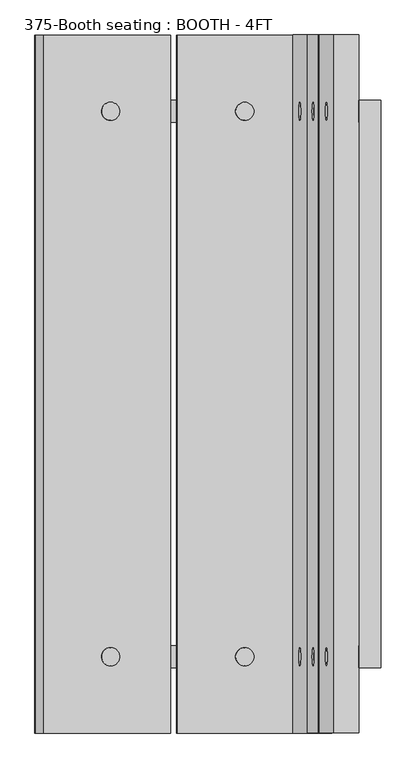
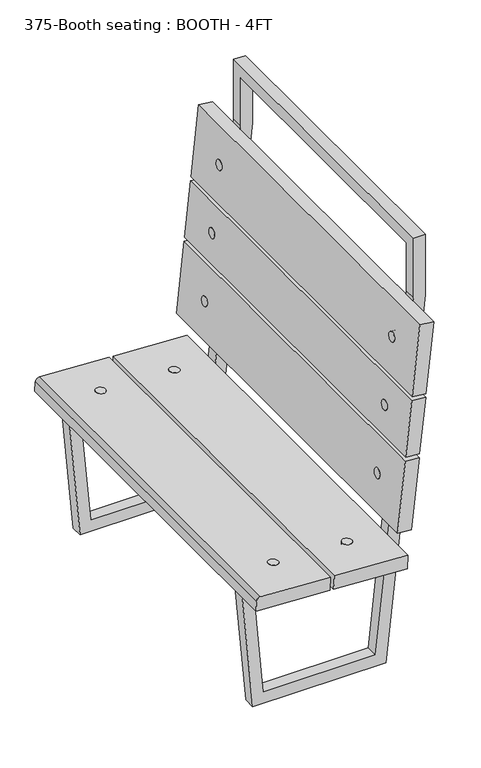
"""IFC4 building model written with IfcOpenShell, lengths in millimetres: furniture geometry, 375-Booth seating : BOOTH - 4FT."""

from ifc_helpers import new_model, si_unit, point, frame, frame_2d, origin, place, context, project, spatial, polyline, circle_curve, trimmed, segment, composite_curve, outline, extrude, faceted_brep, source, transform, mapped, element, save


def furniture_375_booth_seating_booth_4ft_ec9e60ed(model_context):
    return source(origin(), model_context, "Body", "SolidModel", [
        extrude(outline(composite_curve([segment(trimmed(circle_curve(frame_2d((0.0, -15.875)), 15.875), [point((0.0, -31.75))], [point((0.0, 0.0))], False, "CARTESIAN"), True, "CONTINUOUS"), segment(trimmed(circle_curve(frame_2d((0.0, -15.875)), 15.875), [point((0.0, 0.0))], [point((0.0, -31.75))], False, "CARTESIAN"), True, "CONTINUOUS")], self_intersect=False)), frame((476.8022404, 460.375, 403.0070028), z_axis=(0.052335956242943765, 0.0, 0.9986295347545739), x_axis=(-0.9986295347545739, 0.0, 0.052335956242943765)), (0.0, 0.0, 1.0), 44.45),
        extrude(outline(composite_curve([segment(trimmed(circle_curve(frame_2d((-234.95, -15.875)), 15.875), [point((-234.95, -31.75))], [point((-234.95, 0.0))], False, "CARTESIAN"), True, "CONTINUOUS"), segment(trimmed(circle_curve(frame_2d((-234.95, -15.875)), 15.875), [point((-234.95, 0.0))], [point((-234.95, -31.75))], False, "CARTESIAN"), True, "CONTINUOUS")], self_intersect=False)), frame((476.8022404, 460.375, 403.0070028), z_axis=(0.052335956242943765, 0.0, 0.9986295347545739), x_axis=(-0.9986295347545739, 0.0, 0.052335956242943765)), (0.0, 0.0, 1.0), 44.45),
        extrude(outline(composite_curve([segment(trimmed(circle_curve(frame_2d((0.0, 936.625)), 15.875), [point((0.0, 920.75))], [point((0.0, 952.5))], False, "CARTESIAN"), True, "CONTINUOUS"), segment(trimmed(circle_curve(frame_2d((0.0, 936.625)), 15.875), [point((0.0, 952.5))], [point((0.0, 920.75))], False, "CARTESIAN"), True, "CONTINUOUS")], self_intersect=False)), frame((476.8022404, 460.375, 403.0070028), z_axis=(0.052335956242943765, 0.0, 0.9986295347545739), x_axis=(-0.9986295347545739, 0.0, 0.052335956242943765)), (0.0, 0.0, 1.0), 44.45),
        extrude(outline(composite_curve([segment(trimmed(circle_curve(frame_2d((-234.95, 936.625)), 15.875), [point((-234.95, 920.75))], [point((-234.95, 952.5))], False, "CARTESIAN"), True, "CONTINUOUS"), segment(trimmed(circle_curve(frame_2d((-234.95, 936.625)), 15.875), [point((-234.95, 952.5))], [point((-234.95, 920.75))], False, "CARTESIAN"), True, "CONTINUOUS")], self_intersect=False)), frame((476.8022404, 460.375, 403.0070028), z_axis=(0.052335956242943765, 0.0, 0.9986295347545739), x_axis=(-0.9986295347545739, 0.0, 0.052335956242943765)), (0.0, 0.0, 1.0), 44.45),
        extrude(outline(composite_curve([segment(trimmed(circle_curve(frame_2d((0.0, -15.875)), 15.875), [point((0.0, -31.75))], [point((0.0, 0.0))], False, "CARTESIAN"), True, "CONTINUOUS"), segment(trimmed(circle_curve(frame_2d((0.0, -15.875)), 15.875), [point((0.0, 0.0))], [point((0.0, -31.75))], False, "CARTESIAN"), True, "CONTINUOUS")], self_intersect=False)), frame((900.6975371, -492.125, 1069.1522612), z_axis=(-0.9945218953682735, 0.0, 0.10452846326765225), x_axis=(-0.10452846326765225, 0.0, -0.9945218953682735)), (0.0, 0.0, 1.0), 44.45),
        extrude(outline(composite_curve([segment(trimmed(circle_curve(frame_2d((222.2499999, -15.875)), 15.875), [point((222.2499999, -31.75))], [point((222.2499999, 0.0))], False, "CARTESIAN"), True, "CONTINUOUS"), segment(trimmed(circle_curve(frame_2d((222.2499999, -15.875)), 15.875), [point((222.2499999, 0.0))], [point((222.2499999, -31.75))], False, "CARTESIAN"), True, "CONTINUOUS")], self_intersect=False)), frame((900.6975371, -492.125, 1069.1522612), z_axis=(-0.9945218953682735, 0.0, 0.10452846326765225), x_axis=(-0.10452846326765225, 0.0, -0.9945218953682735)), (0.0, 0.0, 1.0), 44.45),
        extrude(outline(composite_curve([segment(trimmed(circle_curve(frame_2d((444.5, -15.875)), 15.875), [point((444.5, -31.75))], [point((444.5, 0.0))], False, "CARTESIAN"), True, "CONTINUOUS"), segment(trimmed(circle_curve(frame_2d((444.5, -15.875)), 15.875), [point((444.5, 0.0))], [point((444.5, -31.75))], False, "CARTESIAN"), True, "CONTINUOUS")], self_intersect=False)), frame((900.6975371, -492.125, 1069.1522612), z_axis=(-0.9945218953682735, 0.0, 0.10452846326765225), x_axis=(-0.10452846326765225, 0.0, -0.9945218953682735)), (0.0, 0.0, 1.0), 44.45),
        extrude(outline(composite_curve([segment(trimmed(circle_curve(frame_2d((0.0, -968.375)), 15.875), [point((0.0, -984.25))], [point((0.0, -952.5))], False, "CARTESIAN"), True, "CONTINUOUS"), segment(trimmed(circle_curve(frame_2d((0.0, -968.375)), 15.875), [point((0.0, -952.5))], [point((0.0, -984.25))], False, "CARTESIAN"), True, "CONTINUOUS")], self_intersect=False)), frame((900.6975371, -492.125, 1069.1522612), z_axis=(-0.9945218953682735, 0.0, 0.10452846326765225), x_axis=(-0.10452846326765225, 0.0, -0.9945218953682735)), (0.0, 0.0, 1.0), 44.45),
        extrude(outline(composite_curve([segment(trimmed(circle_curve(frame_2d((222.2499999, -968.375)), 15.875), [point((222.2499999, -984.25))], [point((222.2499999, -952.5))], False, "CARTESIAN"), True, "CONTINUOUS"), segment(trimmed(circle_curve(frame_2d((222.2499999, -968.375)), 15.875), [point((222.2499999, -952.5))], [point((222.2499999, -984.25))], False, "CARTESIAN"), True, "CONTINUOUS")], self_intersect=False)), frame((900.6975371, -492.125, 1069.1522612), z_axis=(-0.9945218953682735, 0.0, 0.10452846326765225), x_axis=(-0.10452846326765225, 0.0, -0.9945218953682735)), (0.0, 0.0, 1.0), 44.45),
        extrude(outline(composite_curve([segment(trimmed(circle_curve(frame_2d((444.5, -968.375)), 15.875), [point((444.5, -984.25))], [point((444.5, -952.5))], False, "CARTESIAN"), True, "CONTINUOUS"), segment(trimmed(circle_curve(frame_2d((444.5, -968.375)), 15.875), [point((444.5, -952.5))], [point((444.5, -984.25))], False, "CARTESIAN"), True, "CONTINUOUS")], self_intersect=False)), frame((900.6975371, -492.125, 1069.1522612), z_axis=(-0.9945218953682735, 0.0, 0.10452846326765225), x_axis=(-0.10452846326765225, 0.0, -0.9945218953682735)), (0.0, 0.0, 1.0), 44.45),
        faceted_brep([(828.7442542, -457.2, 384.5625035), (914.0084079, -457.2, 1195.7967364), (914.0084079, -457.2, 1358.9), (952.1084079, -457.2, 1358.9), (952.1084079, -457.2, 1193.8), (826.6349718, -457.2, 0.0), (402.5983885, -457.2, 0.0), (366.8356381, -457.2, 408.7701083), (437.5106063, -457.2, 38.1), (792.3295777, -457.2, 38.1), (824.7562543, -457.2, 346.6192193), (408.6106083, -457.2, 368.4284885), (828.7442542, -495.3, 384.5625035), (366.8356381, -495.3, 408.7701083), (402.5983885, -495.3, 0.0), (826.6349718, -495.3, 0.0), (952.1084079, -495.3, 1193.8), (952.1084079, -495.3, 1397.0), (914.0084079, -495.3, 1397.0), (914.0084079, -495.3, 1195.7967364), (437.5106063, -495.3, 38.1), (408.6106083, -495.3, 368.4284885), (824.7562543, -495.3, 346.6192193), (792.3295777, -495.3, 38.1), (914.0084079, 457.2, 1358.9), (952.1084079, 457.2, 1358.9), (828.7442542, 495.3, 384.5625035), (914.0084079, 495.3, 1195.7967364), (914.0084079, 495.3, 1397.0), (952.1084079, 495.3, 1397.0), (952.1084079, 495.3, 1193.8), (826.6349718, 495.3, 0.0), (402.5983885, 495.3, 0.0), (366.8356381, 495.3, 408.7701083), (437.5106063, 495.3, 38.1), (792.3295777, 495.3, 38.1), (824.7562543, 495.3, 346.6192193), (408.6106083, 495.3, 368.4284885), (828.7442542, 457.2, 384.5625035), (366.8356381, 457.2, 408.7701083), (402.5983885, 457.2, 0.0), (826.6349718, 457.2, 0.0), (952.1084079, 457.2, 1193.8), (914.0084079, 457.2, 1195.7967364), (437.5106063, 457.2, 38.1), (408.6106083, 457.2, 368.4284885), (824.7562543, 457.2, 346.6192193), (792.3295777, 457.2, 38.1)], [[[0, 1, 2, 3, 4, 5, 6, 7], [8, 9, 10, 11]], [[12, 13, 14, 15, 16, 17, 18, 19], [20, 21, 22, 23]], [[5, 4, 16, 15]], [[1, 0, 12, 19]], [[0, 7, 13, 12]], [[7, 6, 14, 13]], [[6, 5, 15, 14]], [[8, 11, 21, 20]], [[11, 10, 22, 21]], [[10, 9, 23, 22]], [[9, 8, 20, 23]], [[2, 24, 25, 3]], [[26, 27, 28, 29, 30, 31, 32, 33], [34, 35, 36, 37]], [[38, 39, 40, 41, 42, 25, 24, 43], [44, 45, 46, 47]], [[26, 33, 39, 38]], [[33, 32, 40, 39]], [[32, 31, 41, 40]], [[34, 37, 45, 44]], [[37, 36, 46, 45]], [[36, 35, 47, 46]], [[35, 34, 44, 47]], [[31, 30, 42, 41]], [[27, 26, 38, 43]], [[17, 16, 4, 3, 25, 42, 30, 29]], [[18, 17, 29, 28]], [[19, 18, 28, 27, 43, 24, 2, 1]]]),
        extrude(outline(polyline([(0.0, -44.45), (0.0, 0.0), (1219.2, 0.0), (1219.2, -44.45), (0.0, -44.45)])), frame((841.955154, 609.6, 510.2558191), z_axis=(0.10452846326765272, 0.0, 0.9945218953682734), x_axis=(0.0, -1.0, 0.0)), (0.0, 0.0, 1.0), 234.95),
        extrude(outline(polyline([(0.0, -44.45), (0.0, 0.0), (1219.2, 0.0), (1219.2, -44.45), (0.0, -44.45)])), frame((867.8416279, 609.6, 756.5491664), z_axis=(0.10452846326765385, 0.0, 0.9945218953682733), x_axis=(0.0, -1.0, 0.0)), (0.0, 0.0, 1.0), 184.15),
        extrude(outline(polyline([(0.0, -44.45), (0.0, 0.0), (1219.2, 0.0), (1219.2, -44.45), (0.0, -44.45)])), frame((888.4180559, 609.6, 952.3208015), z_axis=(0.10452846326765004, 0.0, 0.9945218953682737), x_axis=(0.0, -1.0, 0.0)), (0.0, 0.0, 1.0), 234.95),
        extrude(outline(composite_curve([segment(polyline([(441.9125858, 583.7599832), (453.5442521, 361.8145691)]), True, "CONTINUOUS"), segment(trimmed(circle_curve(frame_2d((440.861657, 361.1499024)), 12.7), [point((453.5442521, 361.8145691))], [point((441.5263237, 348.4673073))], False, "CARTESIAN"), True, "CONTINUOUS"), segment(polyline([(441.5263237, 348.4673073), (409.8198359, 346.8056407), (397.4995564, 581.8905778), (441.9125858, 583.7599832)]), True, "CONTINUOUS")], self_intersect=False)), frame((0.0, -609.6, 0.0), z_axis=(0.0, 1.0, 0.0), x_axis=(0.0, 0.0, 1.0)), (0.0, 0.0, 1.0), 1219.2),
        extrude(outline(polyline([(0.0, -234.95), (0.0, 0.0), (1219.2, 0.0), (1219.2, -234.95), (0.0, -234.95)])), frame((828.7442542, 609.6, 384.5625035), z_axis=(0.05233595624294369, 0.0, 0.9986295347545739), x_axis=(0.0, -1.0, 0.0)), (0.0, 0.0, 1.0), 44.45),
    ])


if __name__ == "__main__":
    model = new_model("IFC4")
    model_context = context("Model", 3, world=origin())
    ifc_project = project(units=[si_unit("LENGTHUNIT", "METRE", prefix="MILLI")], contexts=[model_context])
    site = spatial("IfcSite", under=ifc_project)
    building = spatial("IfcBuilding", under=site)
    placement = place(None, origin())
    furniture_375_booth_seating_booth_4ft_shape = furniture_375_booth_seating_booth_4ft_ec9e60ed(model_context)
    element("IfcFurniture", 1, ObjectType="375-Booth seating : BOOTH - 4FT", at=placement, inside=building, context=model_context, shape_type="MappedRepresentation", body=[
        mapped(furniture_375_booth_seating_booth_4ft_shape, transform((0.0, 0.0, 0.0), x_axis=(1.0, 0.0, 0.0), y_axis=(0.0, 1.0, 0.0), z_axis=(0.0, 0.0, 1.0))),
    ])
    save(model, "model.ifc")

# Revit data of these elements
# Type "375-Booth seating : BOOTH - 4FT"
#   tube dim [instance default] = 0' - 1 1/2"
#   seat angle = 3.00°
#   radius of plug = 0' - 0 5/8"
#   plank width_2 = 0' - 7 1/4"
#   plank width_1 = 0' - 9 1/4"
#   plank depth = 0' - 1 3/4"
#   inset = 0' - 6"
#   gap = 0' - 0 1/2"
#   DEPTH = 4' - 0"
#   Seating Count = 2
#   middle support visibility = no
#   Right Bench Visible [instance default] = yes
#   Left Bench Visible [instance default] = yes
#   Material_1 = WOOD-OAKFIRE
#   Material 2 = 1 1/2" SQUARE TUBE STEEL\n- WELDED MITER JOINTS GROUND SMOOTH\n- CLEAR COAT
#   Assembly Code = ""
# Element 1 (IfcFurniture, "375-Booth seating : BOOTH - 4FT")
#   Materials on its faces: "1 1/2\" SQUARE TUBE STEEL\n- WELDED MITER JOINTS GROUND SMOOTH\n- CLEAR COAT", "WOOD-OAKFIRE", "1 1/4\" WOOD PLUG\n(SLIGHTLY DARKER OR STAINED WOOD) - GAL. HEX HEAD THRU BOLT"
# Materials
#   "WOOD-OAKFIRE": class "Wood", colour RGB 198 202 183, transparency 0, Description = "Generic wood", Cost = 0
#   "1 1/2\" SQUARE TUBE STEEL\n- WELDED MITER JOINTS GROUND SMOOTH\n- CLEAR COAT": class "Metal", colour RGB 147 147 147, transparency 0, Cost = 0
#   "1 1/4\" WOOD PLUG\n(SLIGHTLY DARKER OR STAINED WOOD) - GAL. HEX HEAD THRU BOLT": class "Generic", colour RGB 192 192 192, transparency 0, Cost = 0
